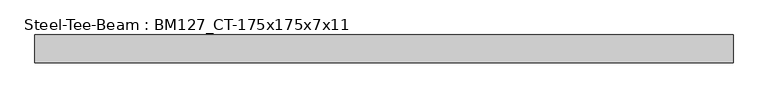
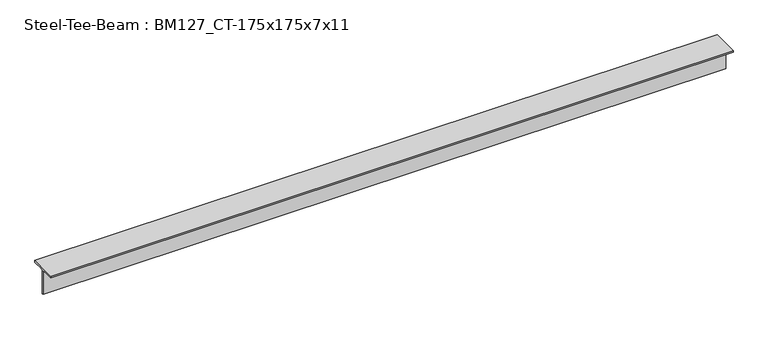
"""IFC4 building model written with IfcOpenShell, lengths in millimetres: beam geometry, Steel-Tee-Beam : BM127_CT-175x175x7x11."""

from ifc_helpers import new_model, si_unit, point, frame, frame_2d, origin, place, context, project, spatial, polyline, circle_curve, trimmed, segment, composite_curve, outline, extrude, source, transform, mapped, element, save


def steel_tee_beam_bm127_ct_175x175x7x11_55b42805(model_context):
    return source(origin(), model_context, "Body", "SweptSolid", [
        extrude(outline(composite_curve([segment(polyline([(-87.5, 87.5), (87.5, 87.5), (87.5, 76.5), (17.5, 76.5)]), True, "CONTINUOUS"), segment(trimmed(circle_curve(frame_2d((17.5, 62.5)), 14.0), [point((17.5, 76.5))], [point((3.5, 62.5))], True, "CARTESIAN"), True, "CONTINUOUS"), segment(polyline([(3.5, 62.5), (3.5, -87.5), (-3.5, -87.5), (-3.5, 62.5)]), True, "CONTINUOUS"), segment(trimmed(circle_curve(frame_2d((-17.5, 62.5)), 14.0), [point((-3.5, 62.5))], [point((-17.5, 76.5))], True, "CARTESIAN"), True, "CONTINUOUS"), segment(polyline([(-17.5, 76.5), (-87.5, 76.5), (-87.5, 87.5)]), True, "CONTINUOUS")], self_intersect=False)), frame((-2195.6471805, 0.0, 0.0), z_axis=(1.0, 0.0, 0.0), x_axis=(0.0, 1.0, 0.0)), (0.0, 0.0, 1.0), 4380.4779119),
    ])


if __name__ == "__main__":
    model = new_model("IFC4")
    model_context = context("Model", 3, world=origin())
    ifc_project = project(units=[si_unit("LENGTHUNIT", "METRE", prefix="MILLI")], contexts=[model_context])
    site = spatial("IfcSite", under=ifc_project)
    building = spatial("IfcBuilding", under=site)
    placement = place(None, origin())
    steel_tee_beam_bm127_ct_175x175x7x11_shape = steel_tee_beam_bm127_ct_175x175x7x11_55b42805(model_context)
    element("IfcBeam", 1, ObjectType="Steel-Tee-Beam : BM127_CT-175x175x7x11", at=placement, inside=building, context=model_context, shape_type="MappedRepresentation", body=[
        mapped(steel_tee_beam_bm127_ct_175x175x7x11_shape, transform((0.0, 0.0, 0.0), x_axis=(1.0, 0.0, 0.0), y_axis=(0.0, 1.0, 0.0), z_axis=(0.0, 0.0, 1.0))),
    ])
    save(model, "model.ifc")

# Revit data of these elements
# Type "Steel-Tee-Beam : BM127_CT-175x175x7x11"
#   Surface Area = 0.00 m²/m
#   Section Area = 31.57 cm²
#   Mass per Unit Length = 24.80 kg/m
#   Length [instance default] = 1524 mm
#   bf = 175 mm
#   d = 175 mm
#   k = 25 mm
#   kr = 14 mm
#   tf = 11 mm
#   tw = 7 mm
#   hec_material4 [instance default] = none
#   hec_material3 [instance default] = none
#   hec_material2 [instance default] = none
#   hec_material1 [instance default] = none
#   Structural Material [instance default] = Steel, 45-345
#   Assembly Code = ""
# Element 1 (IfcBeam, "Steel-Tee-Beam : BM127_CT-175x175x7x11")
#   hec_material3 = F01AC000-00002_Building/Shelter Fire Proofing Work_Intumescent Coating Type_1 hr. rating (UL 1709))
#   hec_material2 = S01AA010-00002_Main Steel Structure Fabrication Work_Shelter/Building_Steel Painting/Coating_for Fireproofed Steel Surface, Surface Preparation & Primer Coat
#   hec_material1 = S03AA029-00001_Main Steel Structure Erection Work_Shelter/Building_Light Steel
#   Structural Material = S01AA003-00001_Main Steel Structure Fabrication Work_Shelter/Building_Light Steel - Standard
#   Materials on its faces: "S01AA003-00001_Main Steel Structure Fabrication Work_Shelter/Building_Light Steel - Standard"
# Materials
#   "Steel, 45-345": class "Metal", colour RGB 189 187 185, transparency 0, Description = "Steel 345 MPa", Cost = 0
#   "S01AA003-00001_Main Steel Structure Fabrication Work_Shelter/Building_Light Steel - Standard": class "Metal", colour RGB 120 120 120, transparency 0, Comments = "(30KG/M>Weight)", Description = "Structural steel 50ksi", W00) Work Master Code = "S01AA003-00001", W01) Work Master_Lv1 = "Main Steel Structure Fabrication Work", W02) Work Master_Lv2 = "Shelter/Building", W03) Work Master_Spec.1 = "Light Steel - Standard (30KG/M>Weight)", Cost = 0
#   "F01AC000-00002_Building/Shelter Fire Proofing Work_Intumescent Coating Type_1 hr. rating (UL 1709))": class "Metal", colour RGB 255 128 128, transparency 0, Description = "Paint finished steel", W00) Work Master Code = "F01AC000-00002", W01) Work Master_Lv1 = "Building/Shelter Fire Proofing Work", W02) Work Master_Lv2 = "Intumescent Coating Type", W03) Work Master_Spec.1 = "1 hr. rating (UL 1709)", Cost = 0
#   "S01AA010-00002_Main Steel Structure Fabrication Work_Shelter/Building_Steel Painting/Coating_for Fireproofed Steel Surface, Surface Preparation & Primer Coat": class "Metal", colour RGB 120 120 120, transparency 0, Description = "Paint finished steel", W00) Work Master Code = "SS01AA010-00002", W01) Work Master_Lv1 = "Main Steel Structure Fabrication Work", W02) Work Master_Lv2 = "Shelter/Building", W03) Work Master_Spec.1 = "Steel Painting/Coating", W04) Work Master_Spec.2 = "for Fireproofed Steel Surface, Surface Preparation & Primer Coat", Cost = 0
#   "S03AA029-00001_Main Steel Structure Erection Work_Shelter/Building_Light Steel": class "Metal", colour RGB 120 120 120, transparency 0, Comments = "(30KG/M>Weight)", Description = "Structural steel 50ksi", W00) Work Master Code = "S03AA029-00001", W01) Work Master_Lv1 = "Main Steel Structure Erection Work", W02) Work Master_Lv2 = "Shelter/Building", W03) Work Master_Spec.1 = "Light Steel (30KG/M>Weight)", Cost = 0
